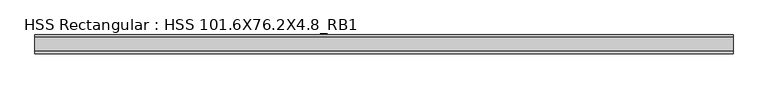
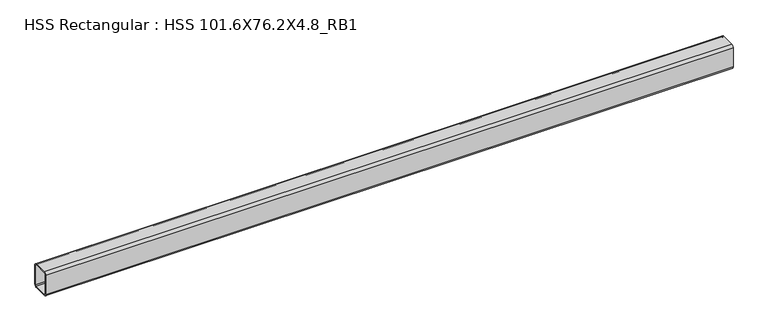
"""IFC4 building model written with IfcOpenShell, lengths in millimetres: beam geometry, HSS Rectangular : HSS 101.6X76.2X4.8_RB1."""

from ifc_helpers import new_model, si_unit, point, frame, frame_2d, origin, place, context, project, spatial, polyline, circle_curve, trimmed, segment, composite_curve, outline, extrude, source, transform, mapped, element, save


def hss_rectangular_hss_101_6x76_2x4_8_rb1_c644dbbb(model_context):
    return source(origin(), model_context, "Body", "SweptSolid", [
        extrude(outline(composite_curve([segment(trimmed(circle_curve(frame_2d((-28.575, 41.275)), 9.525), [point((-38.1, 41.275))], [point((-28.575, 50.8))], False, "CARTESIAN"), True, "CONTINUOUS"), segment(polyline([(-28.575, 50.8), (28.575, 50.8)]), True, "CONTINUOUS"), segment(trimmed(circle_curve(frame_2d((28.575, 41.275)), 9.525), [point((28.575, 50.8))], [point((38.1, 41.275))], False, "CARTESIAN"), True, "CONTINUOUS"), segment(polyline([(38.1, 41.275), (38.1, -41.275)]), True, "CONTINUOUS"), segment(trimmed(circle_curve(frame_2d((28.575, -41.275)), 9.525), [point((38.1, -41.275))], [point((28.575, -50.8))], False, "CARTESIAN"), True, "CONTINUOUS"), segment(polyline([(28.575, -50.8), (-28.575, -50.8)]), True, "CONTINUOUS"), segment(trimmed(circle_curve(frame_2d((-28.575, -41.275)), 9.525), [point((-28.575, -50.8))], [point((-38.1, -41.275))], False, "CARTESIAN"), True, "CONTINUOUS"), segment(polyline([(-38.1, -41.275), (-38.1, 41.275)]), True, "CONTINUOUS")], self_intersect=False), holes=[composite_curve([segment(polyline([(28.575, 46.0375), (-28.575, 46.0375)]), True, "CONTINUOUS"), segment(trimmed(circle_curve(frame_2d((-28.575, 41.275)), 4.7625), [point((-28.575, 46.0375))], [point((-33.3375, 41.275))], True, "CARTESIAN"), True, "CONTINUOUS"), segment(polyline([(-33.3375, 41.275), (-33.3375, -41.275)]), True, "CONTINUOUS"), segment(trimmed(circle_curve(frame_2d((-28.575, -41.275)), 4.7625), [point((-33.3375, -41.275))], [point((-28.575, -46.0375))], True, "CARTESIAN"), True, "CONTINUOUS"), segment(polyline([(-28.575, -46.0375), (28.575, -46.0375)]), True, "CONTINUOUS"), segment(trimmed(circle_curve(frame_2d((28.575, -41.275)), 4.7625), [point((28.575, -46.0375))], [point((33.3375, -41.275))], True, "CARTESIAN"), True, "CONTINUOUS"), segment(polyline([(33.3375, -41.275), (33.3375, 41.275)]), True, "CONTINUOUS"), segment(trimmed(circle_curve(frame_2d((28.575, 41.275)), 4.7625), [point((33.3375, 41.275))], [point((28.575, 46.0375))], True, "CARTESIAN"), True, "CONTINUOUS")], self_intersect=False)]), frame((-1434.0933954, 0.0, 0.0), z_axis=(1.0, 0.0, 0.0), x_axis=(0.0, 1.0, 0.0)), (0.0, 0.0, 1.0), 2811.0367902),
    ])


if __name__ == "__main__":
    model = new_model("IFC4")
    model_context = context("Model", 3, world=origin())
    ifc_project = project(units=[si_unit("LENGTHUNIT", "METRE", prefix="MILLI")], contexts=[model_context])
    site = spatial("IfcSite", under=ifc_project)
    building = spatial("IfcBuilding", under=site)
    placement = place(None, origin())
    hss_rectangular_hss_101_6x76_2x4_8_rb1_shape = hss_rectangular_hss_101_6x76_2x4_8_rb1_c644dbbb(model_context)
    element("IfcBeam", 1, ObjectType="HSS Rectangular : HSS 101.6X76.2X4.8_RB1", at=placement, inside=building, context=model_context, shape_type="MappedRepresentation", body=[
        mapped(hss_rectangular_hss_101_6x76_2x4_8_rb1_shape, transform((0.0, 0.0, 0.0), x_axis=(1.0, 0.0, 0.0), y_axis=(0.0, 1.0, 0.0), z_axis=(0.0, 0.0, 1.0))),
    ])
    save(model, "model.ifc")

# Revit data of these elements
# Type "HSS Rectangular : HSS 101.6X76.2X4.8_RB1"
#   Section Name Key = "HSS 4X3X3/16"
#   Assembly Code = "B10"
#   Width = 7.62 cm
#   Wall Nominal Thickness = 0.4763 cm
#   Wall Design Thickness = 0.442 cm
#   Torsional Moment of Inertia = 260.561 cm⁴
#   Torsional Modulus = 61.2876 cm³
#   Section Area = 14.4516 cm²
#   Plastic Modulus weak axis = 40.3122 cm³
#   Plastic Modulus strong axis = 49.1612 cm³
#   Perimeter = 0.881482 m²/m
#   Outer Fillet = 0.9525 cm
#   Nominal Weight = 12.1285 kgf/m
#   Moment of Inertia weak axis = 131.529 cm⁴
#   Moment of Inertia strong axis = 205.202 cm⁴
#   Inner Fillet = 0.4763 cm
#   Height = 10.16 cm
#   Elastic Modulus weak axis = 34.4128 cm³
#   Elastic Modulus strong axis = 40.476 cm³
#   Centroid Vertical = 5.08 cm
#   Centroid Horizontal = 3.81 cm
#   Length [instance default] = 1524 mm
#   Structural Material [instance default] = Steel ASTM A500, Grade B, Rectangular and Square
#   Principal Axes Angle = 0
# Element 1 (IfcBeam, "HSS Rectangular : HSS 101.6X76.2X4.8_RB1")
#   Structural Material = Steel ASTM A992
#   Materials on its faces: "Steel ASTM A992"
# Materials
#   "Steel ASTM A500, Grade B, Rectangular and Square": class "Metal", colour RGB 199 199 199, transparency 0, Description = "Carbon steel", Cost = 0
#   "Steel ASTM A992": class "Metal", colour RGB 199 199 199, transparency 0, Description = "Structural steel 50ksi", Cost = 0
